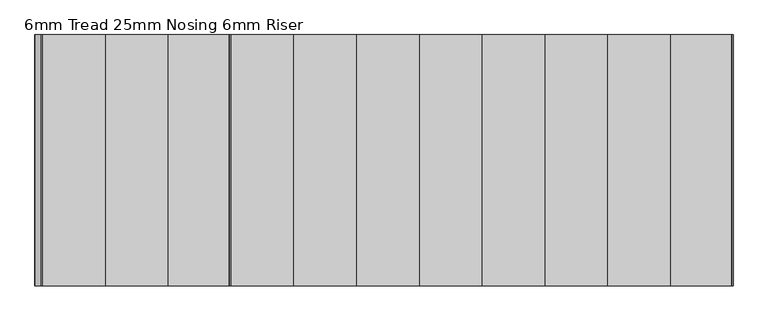
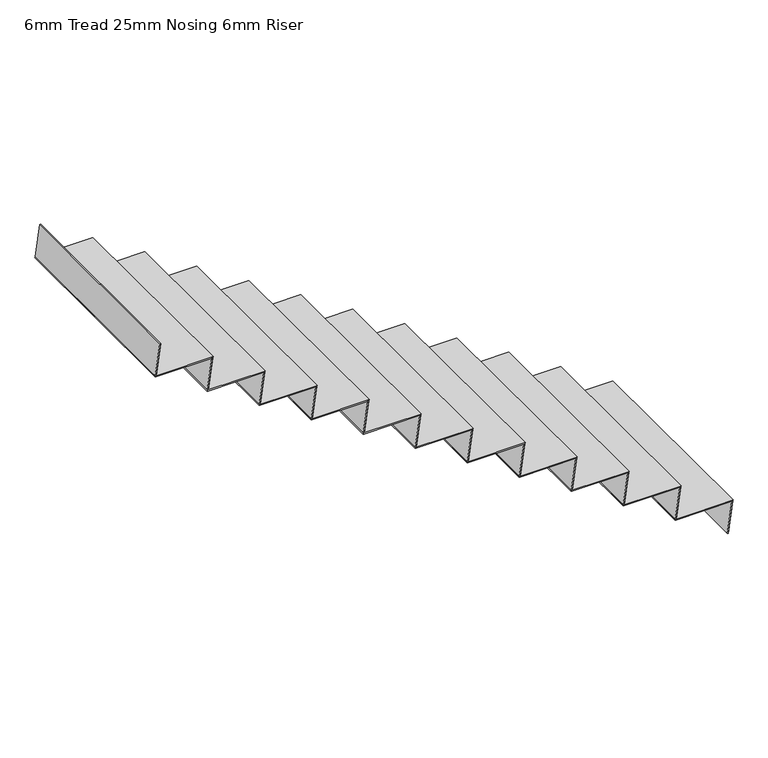
"""IFC4 building model written with IfcOpenShell, lengths in millimetres: stair flight geometry, 6mm Tread 25mm Nosing 6mm Riser."""

from ifc_helpers import new_model, si_unit, origin, place, context, project, spatial, faceted_brep, source, transform, mapped, element, save


def stair_flight_6mm_tread_25mm_nosing_6mm_riser_557edfd0(model_context):
    return source(origin(), model_context, "Body", "Brep", [
        faceted_brep([(-13631.0599092, 11470.4345331, 12235.2941176), (-13631.9099092, 11470.4345331, 12229.2941176), (-13631.9099092, 10370.4345331, 12229.2941176), (-13631.0599092, 10370.4345331, 12235.2941176), (-13325.0, 10370.4345331, 12235.2941176), (-13325.0, 11470.4345331, 12235.2941176), (-13325.85, 11470.4345331, 12229.2941176), (-13325.85, 10370.4345331, 12229.2941176)], [[[0, 1, 2, 3]], [[3, 4, 5, 0]], [[2, 1, 6, 7]], [[4, 3, 2, 7]], [[0, 5, 6, 1]], [[5, 4, 7, 6]]]),
        faceted_brep([(-13325.85, 11470.4345331, 12229.2941176), (-13350.0, 11470.4345331, 12058.8235294), (-13356.0599092, 11470.4345331, 12058.8235294), (-13331.9099092, 11470.4345331, 12229.2941176), (-13325.85, 10370.4345331, 12229.2941176), (-13331.9099092, 10370.4345331, 12229.2941176), (-13356.0599092, 10370.4345331, 12058.8235294), (-13350.0, 10370.4345331, 12058.8235294)], [[[0, 1, 2, 3]], [[4, 5, 6, 7]], [[1, 0, 4, 7]], [[2, 1, 7, 6]], [[3, 2, 6, 5]], [[0, 3, 5, 4]]]),
        faceted_brep([(-13600.85, 11470.4345331, 12405.7647059), (-13625.0, 11470.4345331, 12235.2941176), (-13631.0599092, 11470.4345331, 12235.2941176), (-13606.9099092, 11470.4345331, 12405.7647059), (-13600.85, 10370.4345331, 12405.7647059), (-13606.9099092, 10370.4345331, 12405.7647059), (-13631.0599092, 10370.4345331, 12235.2941176), (-13625.0, 10370.4345331, 12235.2941176)], [[[0, 1, 2, 3]], [[4, 5, 6, 7]], [[1, 0, 4, 7]], [[2, 1, 7, 6]], [[3, 2, 6, 5]], [[0, 3, 5, 4]]]),
        faceted_brep([(-13906.0599092, 10370.4345331, 12411.7647059), (-13600.0, 10370.4345331, 12411.7647059), (-13600.0, 11470.4345331, 12411.7647059), (-13906.0599092, 11470.4345331, 12411.7647059), (-13906.9099092, 10370.4345331, 12405.7647059), (-13906.9099092, 11470.4345331, 12405.7647059), (-13600.85, 11470.4345331, 12405.7647059), (-13600.85, 10370.4345331, 12405.7647059)], [[[0, 1, 2, 3]], [[4, 5, 6, 7]], [[1, 0, 4, 7]], [[3, 2, 6, 5]], [[3, 5, 4, 0]], [[2, 1, 7, 6]]]),
        faceted_brep([(-13875.85, 11470.4345331, 12582.2352941), (-13900.0, 11470.4345331, 12411.7647059), (-13906.0599092, 11470.4345331, 12411.7647059), (-13881.9099092, 11470.4345331, 12582.2352941), (-13875.85, 10370.4345331, 12582.2352941), (-13881.9099092, 10370.4345331, 12582.2352941), (-13906.0599092, 10370.4345331, 12411.7647059), (-13900.0, 10370.4345331, 12411.7647059)], [[[0, 1, 2, 3]], [[4, 5, 6, 7]], [[1, 0, 4, 7]], [[2, 1, 7, 6]], [[3, 2, 6, 5]], [[0, 3, 5, 4]]]),
        faceted_brep([(-14181.0599092, 10370.4345331, 12588.2352941), (-13875.0, 10370.4345331, 12588.2352941), (-13875.0, 11470.4345331, 12588.2352941), (-14181.0599092, 11470.4345331, 12588.2352941), (-14181.9099092, 10370.4345331, 12582.2352941), (-14181.9099092, 11470.4345331, 12582.2352941), (-13875.85, 11470.4345331, 12582.2352941), (-13875.85, 10370.4345331, 12582.2352941)], [[[0, 1, 2, 3]], [[4, 5, 6, 7]], [[1, 0, 4, 7]], [[3, 2, 6, 5]], [[3, 5, 4, 0]], [[2, 1, 7, 6]]]),
        faceted_brep([(-14150.85, 11470.4345331, 12758.7058824), (-14175.0, 11470.4345331, 12588.2352941), (-14181.0599092, 11470.4345331, 12588.2352941), (-14156.9099092, 11470.4345331, 12758.7058824), (-14150.85, 10370.4345331, 12758.7058824), (-14156.9099092, 10370.4345331, 12758.7058824), (-14181.0599092, 10370.4345331, 12588.2352941), (-14175.0, 10370.4345331, 12588.2352941)], [[[0, 1, 2, 3]], [[4, 5, 6, 7]], [[1, 0, 4, 7]], [[2, 1, 7, 6]], [[3, 2, 6, 5]], [[0, 3, 5, 4]]]),
        faceted_brep([(-14456.0599092, 10370.4345331, 12764.7058824), (-14150.0, 10370.4345331, 12764.7058824), (-14150.0, 11470.4345331, 12764.7058824), (-14456.0599092, 11470.4345331, 12764.7058824), (-14456.9099092, 10370.4345331, 12758.7058824), (-14456.9099092, 11470.4345331, 12758.7058824), (-14150.85, 11470.4345331, 12758.7058824), (-14150.85, 10370.4345331, 12758.7058824)], [[[0, 1, 2, 3]], [[4, 5, 6, 7]], [[1, 0, 4, 7]], [[3, 2, 6, 5]], [[3, 5, 4, 0]], [[2, 1, 7, 6]]]),
        faceted_brep([(-14425.85, 11470.4345331, 12935.1764706), (-14450.0, 11470.4345331, 12764.7058824), (-14456.0599092, 11470.4345331, 12764.7058824), (-14431.9099092, 11470.4345331, 12935.1764706), (-14425.85, 10370.4345331, 12935.1764706), (-14431.9099092, 10370.4345331, 12935.1764706), (-14456.0599092, 10370.4345331, 12764.7058824), (-14450.0, 10370.4345331, 12764.7058824)], [[[0, 1, 2, 3]], [[4, 5, 6, 7]], [[1, 0, 4, 7]], [[2, 1, 7, 6]], [[3, 2, 6, 5]], [[0, 3, 5, 4]]]),
        faceted_brep([(-14731.0599092, 10370.4345331, 12941.1764706), (-14425.0, 10370.4345331, 12941.1764706), (-14425.0, 11470.4345331, 12941.1764706), (-14731.0599092, 11470.4345331, 12941.1764706), (-14731.9099092, 10370.4345331, 12935.1764706), (-14731.9099092, 11470.4345331, 12935.1764706), (-14425.85, 11470.4345331, 12935.1764706), (-14425.85, 10370.4345331, 12935.1764706)], [[[0, 1, 2, 3]], [[4, 5, 6, 7]], [[1, 0, 4, 7]], [[3, 2, 6, 5]], [[3, 5, 4, 0]], [[2, 1, 7, 6]]]),
        faceted_brep([(-14700.85, 11470.4345331, 13111.6470588), (-14725.0, 11470.4345331, 12941.1764706), (-14731.0599092, 11470.4345331, 12941.1764706), (-14706.9099092, 11470.4345331, 13111.6470588), (-14700.85, 10370.4345331, 13111.6470588), (-14706.9099092, 10370.4345331, 13111.6470588), (-14731.0599092, 10370.4345331, 12941.1764706), (-14725.0, 10370.4345331, 12941.1764706)], [[[0, 1, 2, 3]], [[4, 5, 6, 7]], [[1, 0, 4, 7]], [[2, 1, 7, 6]], [[3, 2, 6, 5]], [[0, 3, 5, 4]]]),
        faceted_brep([(-15006.0599092, 10370.4345331, 13117.6470588), (-14700.0, 10370.4345331, 13117.6470588), (-14700.0, 11470.4345331, 13117.6470588), (-15006.0599092, 11470.4345331, 13117.6470588), (-15006.9099092, 10370.4345331, 13111.6470588), (-15006.9099092, 11470.4345331, 13111.6470588), (-14700.85, 11470.4345331, 13111.6470588), (-14700.85, 10370.4345331, 13111.6470588)], [[[0, 1, 2, 3]], [[4, 5, 6, 7]], [[1, 0, 4, 7]], [[3, 2, 6, 5]], [[3, 5, 4, 0]], [[2, 1, 7, 6]]]),
        faceted_brep([(-14975.85, 11470.4345331, 13288.1176471), (-15000.0, 11470.4345331, 13117.6470588), (-15006.0599092, 11470.4345331, 13117.6470588), (-14981.9099092, 11470.4345331, 13288.1176471), (-14975.85, 10370.4345331, 13288.1176471), (-14981.9099092, 10370.4345331, 13288.1176471), (-15006.0599092, 10370.4345331, 13117.6470588), (-15000.0, 10370.4345331, 13117.6470588)], [[[0, 1, 2, 3]], [[4, 5, 6, 7]], [[1, 0, 4, 7]], [[2, 1, 7, 6]], [[3, 2, 6, 5]], [[0, 3, 5, 4]]]),
        faceted_brep([(-15281.0599092, 10370.4345331, 13294.1176471), (-14975.0, 10370.4345331, 13294.1176471), (-14975.0, 11470.4345331, 13294.1176471), (-15281.0599092, 11470.4345331, 13294.1176471), (-15281.9099092, 10370.4345331, 13288.1176471), (-15281.9099092, 11470.4345331, 13288.1176471), (-14975.85, 11470.4345331, 13288.1176471), (-14975.85, 10370.4345331, 13288.1176471)], [[[0, 1, 2, 3]], [[4, 5, 6, 7]], [[1, 0, 4, 7]], [[3, 2, 6, 5]], [[3, 5, 4, 0]], [[2, 1, 7, 6]]]),
        faceted_brep([(-15250.85, 11470.4345331, 13464.5882353), (-15275.0, 11470.4345331, 13294.1176471), (-15281.0599092, 11470.4345331, 13294.1176471), (-15256.9099092, 11470.4345331, 13464.5882353), (-15250.85, 10370.4345331, 13464.5882353), (-15256.9099092, 10370.4345331, 13464.5882353), (-15281.0599092, 10370.4345331, 13294.1176471), (-15275.0, 10370.4345331, 13294.1176471)], [[[0, 1, 2, 3]], [[4, 5, 6, 7]], [[1, 0, 4, 7]], [[2, 1, 7, 6]], [[3, 2, 6, 5]], [[0, 3, 5, 4]]]),
        faceted_brep([(-15556.0599092, 10370.4345331, 13470.5882353), (-15250.0, 10370.4345331, 13470.5882353), (-15250.0, 11470.4345331, 13470.5882353), (-15556.0599092, 11470.4345331, 13470.5882353), (-15556.9099092, 10370.4345331, 13464.5882353), (-15556.9099092, 11470.4345331, 13464.5882353), (-15250.85, 11470.4345331, 13464.5882353), (-15250.85, 10370.4345331, 13464.5882353)], [[[0, 1, 2, 3]], [[4, 5, 6, 7]], [[1, 0, 4, 7]], [[3, 2, 6, 5]], [[3, 5, 4, 0]], [[2, 1, 7, 6]]]),
        faceted_brep([(-15525.85, 11470.4345331, 13641.0588235), (-15550.0, 11470.4345331, 13470.5882353), (-15556.0599092, 11470.4345331, 13470.5882353), (-15531.9099092, 11470.4345331, 13641.0588235), (-15525.85, 10370.4345331, 13641.0588235), (-15531.9099092, 10370.4345331, 13641.0588235), (-15556.0599092, 10370.4345331, 13470.5882353), (-15550.0, 10370.4345331, 13470.5882353)], [[[0, 1, 2, 3]], [[4, 5, 6, 7]], [[1, 0, 4, 7]], [[2, 1, 7, 6]], [[3, 2, 6, 5]], [[0, 3, 5, 4]]]),
        faceted_brep([(-15831.0599092, 10370.4345331, 13647.0588235), (-15525.0, 10370.4345331, 13647.0588235), (-15525.0, 11470.4345331, 13647.0588235), (-15831.0599092, 11470.4345331, 13647.0588235), (-15831.9099092, 10370.4345331, 13641.0588235), (-15831.9099092, 11470.4345331, 13641.0588235), (-15525.85, 11470.4345331, 13641.0588235), (-15525.85, 10370.4345331, 13641.0588235)], [[[0, 1, 2, 3]], [[4, 5, 6, 7]], [[1, 0, 4, 7]], [[3, 2, 6, 5]], [[3, 5, 4, 0]], [[2, 1, 7, 6]]]),
        faceted_brep([(-15800.85, 11470.4345331, 13817.5294118), (-15825.0, 11470.4345331, 13647.0588235), (-15831.0599092, 11470.4345331, 13647.0588235), (-15806.9099092, 11470.4345331, 13817.5294118), (-15800.85, 10370.4345331, 13817.5294118), (-15806.9099092, 10370.4345331, 13817.5294118), (-15831.0599092, 10370.4345331, 13647.0588235), (-15825.0, 10370.4345331, 13647.0588235)], [[[0, 1, 2, 3]], [[4, 5, 6, 7]], [[1, 0, 4, 7]], [[2, 1, 7, 6]], [[3, 2, 6, 5]], [[0, 3, 5, 4]]]),
        faceted_brep([(-16106.0599092, 10370.4345331, 13823.5294118), (-15800.0, 10370.4345331, 13823.5294118), (-15800.0, 11470.4345331, 13823.5294118), (-16106.0599092, 11470.4345331, 13823.5294118), (-16106.9099092, 10370.4345331, 13817.5294118), (-16106.9099092, 11470.4345331, 13817.5294118), (-15800.85, 11470.4345331, 13817.5294118), (-15800.85, 10370.4345331, 13817.5294118)], [[[0, 1, 2, 3]], [[4, 5, 6, 7]], [[1, 0, 4, 7]], [[3, 2, 6, 5]], [[3, 5, 4, 0]], [[2, 1, 7, 6]]]),
        faceted_brep([(-16350.85, 11470.4345331, 14170.4705882), (-16375.0, 11470.4345331, 14000.0), (-16381.0599092, 11470.4345331, 14000.0), (-16356.9099092, 11470.4345331, 14170.4705882), (-16350.85, 10370.4345331, 14170.4705882), (-16356.9099092, 10370.4345331, 14170.4705882), (-16381.0599092, 10370.4345331, 14000.0), (-16375.0, 10370.4345331, 14000.0)], [[[0, 1, 2, 3]], [[4, 5, 6, 7]], [[1, 0, 4, 7]], [[2, 1, 7, 6]], [[3, 2, 6, 5]], [[0, 3, 5, 4]]]),
        faceted_brep([(-16075.85, 11470.4345331, 13994.0), (-16100.0, 11470.4345331, 13823.5294118), (-16106.0599092, 11470.4345331, 13823.5294118), (-16081.9099092, 11470.4345331, 13994.0), (-16075.85, 10370.4345331, 13994.0), (-16081.9099092, 10370.4345331, 13994.0), (-16106.0599092, 10370.4345331, 13823.5294118), (-16100.0, 10370.4345331, 13823.5294118)], [[[0, 1, 2, 3]], [[4, 5, 6, 7]], [[1, 0, 4, 7]], [[2, 1, 7, 6]], [[3, 2, 6, 5]], [[0, 3, 5, 4]]]),
        faceted_brep([(-16381.0599092, 10370.4345331, 14000.0), (-16350.0, 10370.4345331, 14000.0), (-16075.0, 10370.4345331, 14000.0), (-16075.0, 11470.4345331, 14000.0), (-16381.0599092, 11470.4345331, 14000.0), (-16381.9099092, 10370.4345331, 13994.0), (-16381.9099092, 11470.4345331, 13994.0), (-16075.85, 11470.4345331, 13994.0), (-16075.85, 10370.4345331, 13994.0), (-16350.0, 10370.4345331, 13994.0)], [[[0, 1, 2, 3, 4]], [[5, 6, 7, 8, 9]], [[1, 0, 5, 9]], [[2, 1, 9, 8]], [[4, 3, 7, 6]], [[4, 6, 5, 0]], [[3, 2, 8, 7]]]),
    ])


if __name__ == "__main__":
    model = new_model("IFC4")
    model_context = context("Model", 3, world=origin())
    ifc_project = project(units=[si_unit("LENGTHUNIT", "METRE", prefix="MILLI")], contexts=[model_context])
    site = spatial("IfcSite", under=ifc_project)
    building = spatial("IfcBuilding", under=site)
    placement = place(None, origin())
    stair_flight_6mm_tread_25mm_nosing_6mm_riser_shape = stair_flight_6mm_tread_25mm_nosing_6mm_riser_557edfd0(model_context)
    element("IfcStairFlight", 1, ObjectType="6mm Tread 25mm Nosing 6mm Riser", at=placement, inside=building, context=model_context, shape_type="MappedRepresentation", body=[
        mapped(stair_flight_6mm_tread_25mm_nosing_6mm_riser_shape, transform((0.0, 0.0, 0.0), x_axis=(1.0, 0.0, 0.0), y_axis=(0.0, 1.0, 0.0), z_axis=(0.0, 0.0, 1.0))),
    ])
    save(model, "model.ifc")

# Revit data of these elements
# Element 1 (IfcStairFlight, "6mm Tread 25mm Nosing 6mm Riser")
#   Materials on its faces: "Steel, Paint Finish, Dark Gray"
# Materials
#   "Steel, Paint Finish, Dark Gray": class "Metal", colour RGB 89 89 89, transparency 0, Description = "Steel, paint finish, dark gray, glossy", Cost = 0
